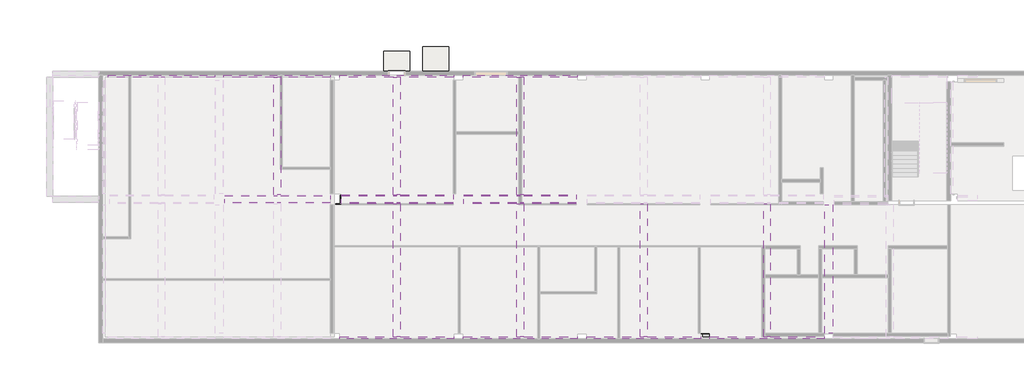
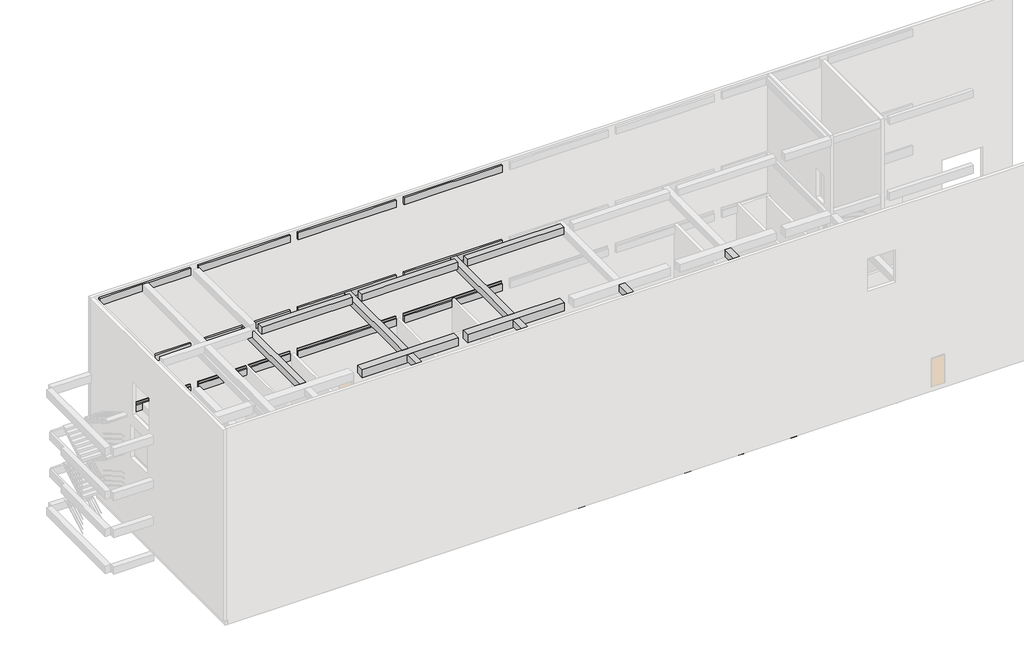
# One storey, part 3 of 5: 54 beams, 2 slabs.
"""IFC4 building model written with IfcOpenShell, lengths in millimetres."""

from ifc_helpers import new_model, si_unit, frame, origin, place, context, project, spatial, polyline, outline, extrude, faceted_brep, element, save

model = new_model("IFC4")

# Units and contexts
model_context = context("Model", 3, world=origin())
ifc_project = project(units=[si_unit("LENGTHUNIT", "METRE", prefix="MILLI")], contexts=[model_context])

# Site, building, storey
site = spatial("IfcSite", under=ifc_project)
building = spatial("IfcBuilding", under=site)
storey = spatial("IfcBuildingStorey", under=building, Name="TOC", Elevation=149.9618634)

# Beams
placement = place(None, origin())
element("IfcBeam", 1, ObjectType="RC Beam_Rectangular : H_SB_AR_S16_UG_B600xH800_1G2", at=placement, inside=storey, context=model_context, shape_type="Brep", body=[
    faceted_brep([(23300.0, 9749.5208589, -550.0381366), (23300.0, 9749.5208589, -150.0381366), (23350.0, 9749.5208589, -150.0381366), (23350.0, 9749.5208589, -0.0381366), (26775.0, 9749.5208589, -0.0381366), (27225.0, 9749.5208589, -0.0381366), (30650.0, 9749.5208589, -0.0381366), (30650.0, 9749.5208589, -150.0381366), (30700.0, 9749.5208589, -150.0381366), (30700.0, 9749.5208589, -550.0381366), (29500.0, 9749.5208589, -550.0381366), (29500.0, 9749.5208589, -650.0381366), (24500.0, 9749.5208589, -650.0381366), (24500.0, 9749.5208589, -550.0381366), (24500.0, 9149.5208589, -650.0381366), (29500.0, 9149.5208589, -650.0381366), (22750.0, 9149.5208589, -550.0381366), (23250.0, 9149.5208589, -550.0381366), (24500.0, 9149.5208589, -550.0381366), (29500.0, 9149.5208589, -550.0381366), (30750.0, 9149.5208589, -550.0381366), (31250.0, 9149.5208589, -550.0381366), (31250.0, 9149.5208589, -150.0381366), (30650.0, 9149.5208589, -150.0381366), (30650.0, 9149.5208589, -0.0381366), (27225.0, 9149.5208589, -0.0381366), (26775.0, 9149.5208589, -0.0381366), (23350.0, 9149.5208589, -0.0381366), (23350.0, 9149.5208589, -150.0381366), (22750.0, 9149.5208589, -150.0381366), (23300.0, 9199.5208589, -550.0381366), (23300.0, 9199.5208589, -150.0381366), (30700.0, 9199.5208589, -150.0381366), (30700.0, 9199.5208589, -550.0381366), (22750.0, 9199.5208589, -550.0381366), (31250.0, 9199.5208589, -550.0381366), (22750.0, 9199.5208589, -150.0381366), (31250.0, 9199.5208589, -150.0381366)], [[[0, 1, 2, 3, 4, 5, 6, 7, 8, 9, 10, 11, 12, 13]], [[14, 12, 11, 15]], [[16, 17, 18, 14, 15, 19, 20, 21, 22, 23, 24, 25, 26, 27, 28, 29]], [[30, 31, 1, 0]], [[32, 33, 9, 8]], [[13, 18, 17, 16, 34, 30, 0]], [[18, 13, 12, 14]], [[19, 10, 9, 33, 35, 21, 20]], [[10, 19, 15, 11]], [[3, 27, 26, 25, 24, 6, 5, 4]], [[31, 30, 34, 36]], [[33, 32, 37, 35]], [[28, 2, 1, 31, 36, 29]], [[2, 28, 27, 3]], [[7, 23, 22, 37, 32, 8]], [[23, 7, 6, 24]], [[36, 34, 16, 29]], [[35, 37, 22, 21]]]),
])
element("IfcBeam", 2, ObjectType="RC Beam_Rectangular : H_SB_AR_S16_UG_B450xH700_1B1", at=placement, inside=storey, context=model_context, shape_type="SweptSolid", body=[
    extrude(outline(polyline([(18775.0, 17399.5208589), (19225.0, 17399.5208589), (19225.0, 9749.5208589), (18775.0, 9749.5208589), (18775.0, 17399.5208589)])), frame((0.0, 0.0, -550.0381366), z_axis=(0.0, 0.0, 1.0), x_axis=(1.0, 0.0, 0.0)), (0.0, 0.0, 1.0), 550.0),
])
element("IfcBeam", 3, ObjectType="RC Beam_Rectangular : H_SB_AR_S16_UG_B450xH700_1B1", at=placement, inside=storey, context=model_context, shape_type="SweptSolid", body=[
    extrude(outline(polyline([(26775.0, 17399.5208589), (27225.0, 17399.5208589), (27225.0, 9749.5208589), (26775.0, 9749.5208589), (26775.0, 17399.5208589)])), frame((0.0, 0.0, -550.0381366), z_axis=(0.0, 0.0, 1.0), x_axis=(1.0, 0.0, 0.0)), (0.0, 0.0, 1.0), 550.0),
])
element("IfcBeam", 4, ObjectType="RC Beam_Rectangular : H_SB_AR_S16_UG_B500xH700_1G1", at=placement, inside=storey, context=model_context, shape_type="SweptSolid", body=[
    extrude(outline(polyline([(9799.5208589, -550.0381366), (9799.5208589, -150.0381366), (9849.5208589, -150.0381366), (9849.5208589, -0.0381366), (17199.5208589, -0.0381366), (17199.5208589, -550.0381366), (9799.5208589, -550.0381366)])), frame((30750.0, 0.0, 0.0), z_axis=(1.0, 0.0, 0.0), x_axis=(0.0, 1.0, 0.0)), (0.0, 0.0, 1.0), 500.0),
])
element("IfcBeam", 5, ObjectType="RC Beam_Rectangular : H_SB_AR_S16_UG_B500xH700_1G1", at=placement, inside=storey, context=model_context, shape_type="SweptSolid", body=[
    extrude(outline(polyline([(17199.5208589, -0.0381366), (17199.5208589, -550.0381366), (9799.5208589, -550.0381366), (9799.5208589, -150.0381366), (9849.5208589, -150.0381366), (9849.5208589, -0.0381366), (17199.5208589, -0.0381366)])), frame((22750.0, 0.0, 0.0), z_axis=(1.0, 0.0, 0.0), x_axis=(0.0, 1.0, 0.0)), (0.0, 0.0, 1.0), 500.0),
])
element("IfcBeam", 6, ObjectType="RC Beam_Rectangular : H_SB_AR_S16_UG_B500xH700_1G1", at=placement, inside=storey, context=model_context, shape_type="Brep", body=[
    faceted_brep([(23250.0, 9149.5208589, -550.0381366), (22750.0, 9149.5208589, -550.0381366), (22750.0, 9149.5208589, -150.0381366), (22750.0, 9149.5208589, -0.0381366), (23250.0, 9149.5208589, -0.0381366), (22750.0, 799.5208589, -550.0381366), (22750.0, 799.5208589, -0.0381366), (23250.0, 799.5208589, -550.0381366), (23250.0, 799.5208589, -0.0381366)], [[[0, 1, 2, 3, 4]], [[5, 6, 3, 2, 1]], [[1, 0, 7, 5]], [[8, 7, 0, 4]], [[5, 7, 8, 6]], [[3, 6, 8, 4]]]),
])
element("IfcBeam", 7, ObjectType="RC Beam_Rectangular : H_SB_AR_S16_UG_B500xH700_1G1", at=placement, inside=storey, context=model_context, shape_type="Brep", body=[
    faceted_brep([(30750.0, 799.5208589, -550.0381366), (30750.0, 799.5208589, -0.0381366), (30750.0, 9149.5208589, -0.0381366), (30750.0, 9149.5208589, -550.0381366), (31250.0, 799.5208589, -550.0381366), (31250.0, 9149.5208589, -550.0381366), (31250.0, 799.5208589, -0.0381366), (31250.0, 9149.5208589, -150.0381366), (31250.0, 9149.5208589, -0.0381366)], [[[0, 1, 2, 3]], [[4, 0, 3, 5]], [[6, 4, 5, 7, 8]], [[0, 4, 6, 1]], [[2, 1, 6, 8]], [[5, 3, 2, 8, 7]]]),
])
element("IfcBeam", 8, ObjectType="RC Beam_Rectangular : H_SB_AR_S16_UG_B500xH700_1G1", at=placement, inside=storey, context=model_context, shape_type="Brep", body=[
    faceted_brep([(39249.6103984, 9148.7405199, -550.0381366), (38749.610707, 9149.2960751, -550.0381366), (38749.610707, 9149.2960751, -0.0381366), (39249.6103984, 9148.7405199, -0.0381366), (39240.3344102, 800.351107, 149.9618634), (38740.3341015, 800.351107, 149.9618634), (38740.333179, 799.5208589, 149.9618634), (39240.3334877, 799.5208589, 149.9618634), (38740.333179, 799.5208589, -550.0381366), (38740.3341015, 800.351107, -0.0381366), (39240.1112654, 599.5208589, -550.0381366), (38850.0, 599.5208589, -550.0381366), (38850.0, 799.5208589, -550.0381366), (39240.3344102, 800.351107, -0.0381366), (39240.3334877, 799.5208589, -150.0381366), (39240.1112654, 599.5208589, -150.0381366), (38850.0, 799.5208589, -150.0381366), (38850.0, 599.5208589, -150.0381366)], [[[0, 1, 2, 3]], [[4, 5, 6, 7]], [[8, 6, 5, 9, 2, 1]], [[1, 0, 10, 11, 12, 8]], [[3, 13, 4, 7, 14, 15, 10, 0]], [[8, 12, 16, 14, 7, 6]], [[2, 9, 13, 3]], [[5, 4, 13, 9]], [[11, 10, 15, 17]], [[14, 16, 17, 15]], [[16, 12, 11, 17]]]),
])
element("IfcBeam", 9, ObjectType="RC Beam_Rectangular : H_SB_AR_S16_UG_B500xH700_1G1", at=placement, inside=storey, context=model_context, shape_type="Brep", body=[
    faceted_brep([(46750.0, 799.5208589, -550.0381366), (46750.0, 799.5208589, -0.0381366), (46750.0, 9149.5208589, -0.0381366), (46750.0, 9149.5208589, -550.0381366), (47250.0, 799.5208589, -550.0381366), (47250.0, 9149.5208589, -550.0381366), (47250.0, 799.5208589, -0.0381366), (47250.0, 9149.5208589, -150.0381366), (47250.0, 9149.5208589, -0.0381366)], [[[0, 1, 2, 3]], [[4, 0, 3, 5]], [[6, 4, 5, 7, 8]], [[0, 4, 6, 1]], [[2, 1, 6, 8]], [[2, 8, 7, 5, 3]]]),
])
element("IfcBeam", 10, ObjectType="RC Beam_Rectangular : H_SB_AR_S16_UG_B450xH700_1B1A", at=placement, inside=storey, context=model_context, shape_type="SweptSolid", body=[
    extrude(outline(polyline([(43225.0, 599.5208589), (42775.0, 599.5208589), (42775.0, 9149.5208589), (43225.0, 9149.5208589), (43225.0, 599.5208589)])), frame((0.0, 0.0, -550.0381366), z_axis=(0.0, 0.0, 1.0), x_axis=(1.0, 0.0, 0.0)), (0.0, 0.0, 1.0), 550.0),
])
element("IfcBeam", 11, ObjectType="RC Beam_Rectangular : H_SB_AR_S16_UG_B450xH700_1B1A", at=placement, inside=storey, context=model_context, shape_type="SweptSolid", body=[
    extrude(outline(polyline([(35225.0, 599.5208589), (34775.0, 599.5208589), (34775.0, 9149.5208589), (35225.0, 9149.5208589), (35225.0, 599.5208589)])), frame((0.0, 0.0, -550.0381366), z_axis=(0.0, 0.0, 1.0), x_axis=(1.0, 0.0, 0.0)), (0.0, 0.0, 1.0), 550.0),
])
element("IfcBeam", 12, ObjectType="RC Beam_Rectangular : H_SB_AR_S16_UG_B450xH700_1B1A", at=placement, inside=storey, context=model_context, shape_type="SweptSolid", body=[
    extrude(outline(polyline([(27225.0, 599.5208589), (26775.0, 599.5208589), (26775.0, 9149.5208589), (27225.0, 9149.5208589), (27225.0, 599.5208589)])), frame((0.0, 0.0, -550.0381366), z_axis=(0.0, 0.0, 1.0), x_axis=(1.0, 0.0, 0.0)), (0.0, 0.0, 1.0), 550.0),
])
element("IfcBeam", 13, ObjectType="RC Beam_Rectangular : H_SB_AR_S16_UG_B450xH700_1B1A", at=placement, inside=storey, context=model_context, shape_type="SweptSolid", body=[
    extrude(outline(polyline([(19225.0, 599.5208589), (18775.0, 599.5208589), (18775.0, 9149.5208589), (19225.0, 9149.5208589), (19225.0, 599.5208589)])), frame((0.0, 0.0, -550.0381366), z_axis=(0.0, 0.0, 1.0), x_axis=(1.0, 0.0, 0.0)), (0.0, 0.0, 1.0), 550.0),
])
element("IfcBeam", 14, ObjectType="RC Beam_Rectangular : H_SB_AR_S16_AG_B400xH700_3WG1", at=placement, inside=storey, context=model_context, shape_type="Brep", body=[
    faceted_brep([(300.0, 17499.5208589, 5949.9618634), (7200.0, 17499.5208589, 5949.9618634), (7200.0, 17549.5208589, 5949.9618634), (300.0, 17549.5208589, 5949.9618634), (300.0, 17399.5208589, 5799.9618634), (300.0, 17399.5208589, 5249.9618634), (3525.0, 17399.5208589, 5249.9618634), (3975.0, 17399.5208589, 5249.9618634), (7200.0, 17399.5208589, 5249.9618634), (7200.0, 17399.5208589, 5799.9618634), (3975.0, 17399.5208589, 5799.9618634), (3525.0, 17399.5208589, 5799.9618634), (300.0, 17549.5208589, 5249.9618634), (7200.0, 17549.5208589, 5249.9618634), (300.0, 17499.5208589, 5799.9618634), (7200.0, 17499.5208589, 5799.9618634)], [[[0, 1, 2, 3]], [[4, 5, 6, 7, 8, 9, 10, 11]], [[8, 7, 6, 5, 12, 13]], [[14, 4, 11, 10, 9, 15]], [[0, 14, 15, 1]], [[5, 4, 14, 0, 3, 12]], [[9, 8, 13, 2, 1, 15]], [[3, 2, 13, 12]]]),
])
element("IfcBeam", 15, ObjectType="RC Beam_Rectangular : H_SB_AR_S16_AG_B400xH700_3WG1", at=placement, inside=storey, context=model_context, shape_type="Brep", body=[
    faceted_brep([(7800.0, 17499.5208589, 5949.9618634), (14700.0, 17499.5208589, 5949.9618634), (14700.0, 17549.5208589, 5949.9618634), (7800.0, 17549.5208589, 5949.9618634), (7800.0, 17399.5208589, 5799.9618634), (7800.0, 17399.5208589, 5249.9618634), (11050.0, 17399.5208589, 5249.9618634), (11500.0, 17399.5208589, 5249.9618634), (14700.0, 17399.5208589, 5249.9618634), (14700.0, 17399.5208589, 5799.9618634), (11500.0, 17399.5208589, 5799.9618634), (11050.0, 17399.5208589, 5799.9618634), (7800.0, 17549.5208589, 5249.9618634), (14700.0, 17549.5208589, 5249.9618634), (7800.0, 17499.5208589, 5799.9618634), (14700.0, 17499.5208589, 5799.9618634)], [[[0, 1, 2, 3]], [[4, 5, 6, 7, 8, 9, 10, 11]], [[8, 7, 6, 5, 12, 13]], [[14, 4, 11, 10, 9, 15]], [[0, 14, 15, 1]], [[5, 4, 14, 0, 3, 12]], [[9, 8, 13, 2, 1, 15]], [[3, 2, 13, 12]]]),
])
element("IfcBeam", 16, ObjectType="RC Beam_Rectangular : H_SB_AR_S16_AG_B400xH700_3WG1", at=placement, inside=storey, context=model_context, shape_type="Brep", body=[
    faceted_brep([(15300.0, 17499.5208589, 5949.9618634), (22700.0, 17499.5208589, 5949.9618634), (22700.0, 17549.5208589, 5949.9618634), (15300.0, 17549.5208589, 5949.9618634), (15300.0, 17399.5208589, 5799.9618634), (15300.0, 17399.5208589, 5249.9618634), (18800.0, 17399.5208589, 5249.9618634), (19250.0, 17399.5208589, 5249.9618634), (22700.0, 17399.5208589, 5249.9618634), (22700.0, 17399.5208589, 5799.9618634), (19250.0, 17399.5208589, 5799.9618634), (18800.0, 17399.5208589, 5799.9618634), (15300.0, 17549.5208589, 5249.9618634), (22700.0, 17549.5208589, 5249.9618634), (15300.0, 17499.5208589, 5799.9618634), (22700.0, 17499.5208589, 5799.9618634)], [[[0, 1, 2, 3]], [[4, 5, 6, 7, 8, 9, 10, 11]], [[8, 7, 6, 5, 12, 13]], [[14, 4, 11, 10, 9, 15]], [[0, 14, 15, 1]], [[5, 4, 14, 0, 3, 12]], [[9, 8, 13, 2, 1, 15]], [[3, 2, 13, 12]]]),
])
element("IfcBeam", 17, ObjectType="RC Beam_Rectangular : H_SB_AR_S16_AG_B400xH700_3WG1", at=placement, inside=storey, context=model_context, shape_type="Brep", body=[
    faceted_brep([(23300.0, 17499.5208589, 5949.9618634), (30700.0, 17499.5208589, 5949.9618634), (30700.0, 17549.5208589, 5949.9618634), (23300.0, 17549.5208589, 5949.9618634), (23300.0, 17399.5208589, 5799.9618634), (23300.0, 17399.5208589, 5249.9618634), (26775.0, 17399.5208589, 5249.9618634), (27225.0, 17399.5208589, 5249.9618634), (30700.0, 17399.5208589, 5249.9618634), (30700.0, 17399.5208589, 5799.9618634), (27225.0, 17399.5208589, 5799.9618634), (26775.0, 17399.5208589, 5799.9618634), (23300.0, 17549.5208589, 5249.9618634), (30700.0, 17549.5208589, 5249.9618634), (23300.0, 17499.5208589, 5799.9618634), (30700.0, 17499.5208589, 5799.9618634)], [[[0, 1, 2, 3]], [[4, 5, 6, 7, 8, 9, 10, 11]], [[8, 7, 6, 5, 12, 13]], [[14, 4, 11, 10, 9, 15]], [[0, 14, 15, 1]], [[5, 4, 14, 0, 3, 12]], [[9, 8, 13, 2, 1, 15]], [[3, 2, 13, 12]]]),
])
element("IfcBeam", 18, ObjectType="RC Beam_Rectangular : H_SB_AR_S16_AG_B400xH700_3WG1", at=placement, inside=storey, context=model_context, shape_type="Brep", body=[
    faceted_brep([(22700.0, 449.5208589, 5949.9618634), (22700.0, 499.5208589, 5949.9618634), (15300.0, 499.5208589, 5949.9618634), (15300.0, 449.5208589, 5949.9618634), (22700.0, 599.5208589, 5249.9618634), (22700.0, 449.5208589, 5249.9618634), (15300.0, 449.5208589, 5249.9618634), (15300.0, 599.5208589, 5249.9618634), (18785.0, 599.5208589, 5249.9618634), (19235.0, 599.5208589, 5249.9618634), (22700.0, 599.5208589, 5799.9618634), (15300.0, 599.5208589, 5799.9618634), (18785.0, 599.5208589, 5799.9618634), (19235.0, 599.5208589, 5799.9618634), (22700.0, 499.5208589, 5799.9618634), (15300.0, 499.5208589, 5799.9618634)], [[[0, 1, 2, 3]], [[4, 5, 6, 7, 8, 9]], [[10, 4, 9, 8, 7, 11, 12, 13]], [[5, 0, 3, 6]], [[14, 10, 13, 12, 11, 15]], [[1, 14, 15, 2]], [[1, 0, 5, 4, 10, 14]], [[3, 2, 15, 11, 7, 6]]]),
])
element("IfcBeam", 19, ObjectType="RC Beam_Rectangular : H_SB_AR_S16_AG_B400xH700_3WG1", at=placement, inside=storey, context=model_context, shape_type="Brep", body=[
    faceted_brep([(30700.0, 449.5208589, 5949.9618634), (30700.0, 499.5208589, 5949.9618634), (23300.0, 499.5208589, 5949.9618634), (23300.0, 449.5208589, 5949.9618634), (30700.0, 599.5208589, 5249.9618634), (30700.0, 449.5208589, 5249.9618634), (23300.0, 449.5208589, 5249.9618634), (23300.0, 599.5208589, 5249.9618634), (26785.0, 599.5208589, 5249.9618634), (27235.0, 599.5208589, 5249.9618634), (30700.0, 599.5208589, 5799.9618634), (23300.0, 599.5208589, 5799.9618634), (26785.0, 599.5208589, 5799.9618634), (27235.0, 599.5208589, 5799.9618634), (30700.0, 499.5208589, 5799.9618634), (23300.0, 499.5208589, 5799.9618634)], [[[0, 1, 2, 3]], [[4, 5, 6, 7, 8, 9]], [[10, 4, 9, 8, 7, 11, 12, 13]], [[5, 0, 3, 6]], [[14, 10, 13, 12, 11, 15]], [[1, 14, 15, 2]], [[1, 0, 5, 4, 10, 14]], [[3, 2, 15, 11, 7, 6]]]),
])
element("IfcBeam", 20, ObjectType="RC Beam_Rectangular : H_SB_AR_S16_AG_B400xH700_3WG1", at=placement, inside=storey, context=model_context, shape_type="Brep", body=[
    faceted_brep([(38700.0, 449.5208589, 5949.9618634), (38700.0, 499.5208589, 5949.9618634), (31300.0, 499.5208589, 5949.9618634), (31300.0, 449.5208589, 5949.9618634), (38700.0, 599.5208589, 5249.9618634), (38700.0, 449.5208589, 5249.9618634), (31300.0, 449.5208589, 5249.9618634), (31300.0, 599.5208589, 5249.9618634), (34785.0, 599.5208589, 5249.9618634), (35235.0, 599.5208589, 5249.9618634), (38700.0, 599.5208589, 5799.9618634), (31300.0, 599.5208589, 5799.9618634), (34785.0, 599.5208589, 5799.9618634), (35235.0, 599.5208589, 5799.9618634), (38700.0, 499.5208589, 5799.9618634), (31300.0, 499.5208589, 5799.9618634)], [[[0, 1, 2, 3]], [[4, 5, 6, 7, 8, 9]], [[10, 4, 9, 8, 7, 11, 12, 13]], [[5, 0, 3, 6]], [[14, 10, 13, 12, 11, 15]], [[1, 14, 15, 2]], [[1, 0, 5, 4, 10, 14]], [[3, 2, 15, 11, 7, 6]]]),
])
element("IfcBeam", 21, ObjectType="RC Beam_Rectangular : H_SB_AR_S16_AG_B400xH700_3WG1", at=placement, inside=storey, context=model_context, shape_type="Brep", body=[
    faceted_brep([(46700.0, 449.5208589, 5949.9618634), (46700.0, 499.5208589, 5949.9618634), (39300.0, 499.5208589, 5949.9618634), (39300.0, 449.5208589, 5949.9618634), (46700.0, 599.5208589, 5249.9618634), (46700.0, 449.5208589, 5249.9618634), (39300.0, 449.5208589, 5249.9618634), (39300.0, 599.5208589, 5249.9618634), (42785.0, 599.5208589, 5249.9618634), (43235.0, 599.5208589, 5249.9618634), (46700.0, 599.5208589, 5799.9618634), (39300.0, 599.5208589, 5799.9618634), (42785.0, 599.5208589, 5799.9618634), (43235.0, 599.5208589, 5799.9618634), (46700.0, 499.5208589, 5799.9618634), (39300.0, 499.5208589, 5799.9618634)], [[[0, 1, 2, 3]], [[4, 5, 6, 7, 8, 9]], [[10, 4, 9, 8, 7, 11, 12, 13]], [[5, 0, 3, 6]], [[14, 10, 13, 12, 11, 15]], [[1, 14, 15, 2]], [[1, 0, 5, 4, 10, 14]], [[3, 2, 15, 11, 7, 6]]]),
])
element("IfcBeam", 22, ObjectType="RC Beam_Rectangular : H_SB_AR_S16_AG_B600xH800_3G2", at=placement, inside=storey, context=model_context, shape_type="Brep", body=[
    faceted_brep([(15400.0, 9199.5208589, 5149.9618634), (22650.0, 9199.5208589, 5149.9618634), (22650.0, 9199.5208589, 5799.9618634), (19235.0, 9199.5208589, 5799.9618634), (18785.0, 9199.5208589, 5799.9618634), (15400.0, 9199.5208589, 5799.9618634), (15400.0, 9799.5208589, 5149.9618634), (22650.0, 9799.5208589, 5149.9618634), (15400.0, 9799.5208589, 5799.9618634), (18800.0, 9799.5208589, 5799.9618634), (19250.0, 9799.5208589, 5799.9618634), (22650.0, 9799.5208589, 5799.9618634)], [[[0, 1, 2, 3, 4, 5]], [[1, 0, 6, 7]], [[7, 6, 8, 9, 10, 11]], [[5, 4, 3, 2, 11, 10, 9, 8]], [[1, 7, 11, 2]], [[6, 0, 5, 8]]]),
])
element("IfcBeam", 23, ObjectType="RC Beam_Rectangular : H_SB_AR_S16_AG_B600xH800_3G2", at=placement, inside=storey, context=model_context, shape_type="Brep", body=[
    faceted_brep([(23350.0, 9199.5208589, 5149.9618634), (30650.0, 9199.5208589, 5149.9618634), (30650.0, 9199.5208589, 5799.9618634), (27235.0, 9199.5208589, 5799.9618634), (26785.0, 9199.5208589, 5799.9618634), (23350.0, 9199.5208589, 5799.9618634), (23350.0, 9799.5208589, 5149.9618634), (30650.0, 9799.5208589, 5149.9618634), (23350.0, 9799.5208589, 5799.9618634), (26775.0, 9799.5208589, 5799.9618634), (27225.0, 9799.5208589, 5799.9618634), (30650.0, 9799.5208589, 5799.9618634)], [[[0, 1, 2, 3, 4, 5]], [[1, 0, 6, 7]], [[7, 6, 8, 9, 10, 11]], [[5, 4, 3, 2, 11, 10, 9, 8]], [[6, 0, 5, 8]], [[1, 7, 11, 2]]]),
])
element("IfcBeam", 24, ObjectType="RC Beam_Rectangular : H_SB_AR_S16_AG_B4500xH700_3G1", at=placement, inside=storey, context=model_context, shape_type="SweptSolid", body=[
    extrude(outline(polyline([(46750.0, 799.5208589), (46750.0, 9149.5208589), (47250.0, 9149.5208589), (47250.0, 799.5208589), (46750.0, 799.5208589)])), frame((0.0, 0.0, 5249.9618634), z_axis=(0.0, 0.0, 1.0), x_axis=(1.0, 0.0, 0.0)), (0.0, 0.0, 1.0), 550.0),
])
element("IfcBeam", 25, ObjectType="RC Beam_Rectangular : H_SB_AR_S16_AG_B400xH700_3WG1", at=placement, inside=storey, context=model_context, shape_type="Brep", body=[
    faceted_brep([(300.0, 17399.5208589, 9269.9618634), (300.0, 17399.5208589, 8749.9618634), (3525.0, 17399.5208589, 8749.9618634), (3975.0, 17399.5208589, 8749.9618634), (7200.0, 17399.5208589, 8749.9618634), (7200.0, 17399.5208589, 9269.9618634), (3975.0, 17399.5208589, 9269.9618634), (3525.0, 17399.5208589, 9269.9618634), (300.0, 17549.5208589, 8749.9618634), (7200.0, 17549.5208589, 8749.9618634), (300.0, 17549.5208589, 9269.9618634), (7200.0, 17549.5208589, 9269.9618634)], [[[0, 1, 2, 3, 4, 5, 6, 7]], [[4, 3, 2, 1, 8, 9]], [[10, 0, 7, 6, 5, 11]], [[1, 0, 10, 8]], [[5, 4, 9, 11]], [[9, 8, 10, 11]]]),
])
element("IfcBeam", 26, ObjectType="RC Beam_Rectangular : H_SB_AR_S16_AG_B400xH700_3WG1", at=placement, inside=storey, context=model_context, shape_type="Brep", body=[
    faceted_brep([(7800.0, 17399.5208589, 9269.9618634), (7800.0, 17399.5208589, 8749.9618634), (11025.0, 17399.5208589, 8749.9618634), (11475.0, 17399.5208589, 8749.9618634), (14700.0, 17399.5208589, 8749.9618634), (14700.0, 17399.5208589, 9269.9618634), (11475.0, 17399.5208589, 9269.9618634), (11025.0, 17399.5208589, 9269.9618634), (7800.0, 17549.5208589, 8749.9618634), (14700.0, 17549.5208589, 8749.9618634), (7800.0, 17549.5208589, 9269.9618634), (14700.0, 17549.5208589, 9269.9618634)], [[[0, 1, 2, 3, 4, 5, 6, 7]], [[4, 3, 2, 1, 8, 9]], [[10, 0, 7, 6, 5, 11]], [[1, 0, 10, 8]], [[5, 4, 9, 11]], [[9, 8, 10, 11]]]),
])
element("IfcBeam", 27, ObjectType="RC Beam_Rectangular : H_SB_AR_S16_AG_B400xH700_3WG1", at=placement, inside=storey, context=model_context, shape_type="Brep", body=[
    faceted_brep([(15300.0, 17399.5208589, 9269.9618634), (15300.0, 17399.5208589, 8749.9618634), (18775.0, 17399.5208589, 8749.9618634), (19225.0, 17399.5208589, 8749.9618634), (22700.0, 17399.5208589, 8749.9618634), (22700.0, 17399.5208589, 9269.9618634), (19225.0, 17399.5208589, 9269.9618634), (18775.0, 17399.5208589, 9269.9618634), (15300.0, 17549.5208589, 8749.9618634), (22700.0, 17549.5208589, 8749.9618634), (15300.0, 17549.5208589, 9269.9618634), (22700.0, 17549.5208589, 9269.9618634)], [[[0, 1, 2, 3, 4, 5, 6, 7]], [[4, 3, 2, 1, 8, 9]], [[10, 0, 7, 6, 5, 11]], [[1, 0, 10, 8]], [[5, 4, 9, 11]], [[9, 8, 10, 11]]]),
])
element("IfcBeam", 28, ObjectType="RC Beam_Rectangular : H_SB_AR_S16_AG_B400xH700_3WG1", at=placement, inside=storey, context=model_context, shape_type="Brep", body=[
    faceted_brep([(23300.0, 17399.5208589, 9269.9618634), (23300.0, 17399.5208589, 8749.9618634), (26775.0, 17399.5208589, 8749.9618634), (27225.0, 17399.5208589, 8749.9618634), (30700.0, 17399.5208589, 8749.9618634), (30700.0, 17399.5208589, 9269.9618634), (27225.0, 17399.5208589, 9269.9618634), (26775.0, 17399.5208589, 9269.9618634), (23300.0, 17549.5208589, 8749.9618634), (30700.0, 17549.5208589, 8749.9618634), (23300.0, 17549.5208589, 9269.9618634), (30700.0, 17549.5208589, 9269.9618634)], [[[0, 1, 2, 3, 4, 5, 6, 7]], [[4, 3, 2, 1, 8, 9]], [[10, 0, 7, 6, 5, 11]], [[1, 0, 10, 8]], [[5, 4, 9, 11]], [[9, 8, 10, 11]]]),
])
element("IfcBeam", 29, ObjectType="RC Beam_Rectangular : H_SB_AR_S16_AG_B400xH700_3WG1", at=placement, inside=storey, context=model_context, shape_type="Brep", body=[
    faceted_brep([(22700.0, 599.5208589, 8749.9618634), (22700.0, 449.5208589, 8749.9618634), (15300.0, 449.5208589, 8749.9618634), (15300.0, 599.5208589, 8749.9618634), (18775.0, 599.5208589, 8749.9618634), (19225.0, 599.5208589, 8749.9618634), (22700.0, 599.5208589, 9269.9618634), (15300.0, 599.5208589, 9269.9618634), (18775.0, 599.5208589, 9269.9618634), (19225.0, 599.5208589, 9269.9618634), (22700.0, 449.5208589, 9269.9618634), (15300.0, 449.5208589, 9269.9618634)], [[[0, 1, 2, 3, 4, 5]], [[6, 0, 5, 4, 3, 7, 8, 9]], [[1, 10, 11, 2]], [[10, 6, 9, 8, 7, 11]], [[1, 0, 6, 10]], [[3, 2, 11, 7]]]),
])
element("IfcBeam", 30, ObjectType="RC Beam_Rectangular : H_SB_AR_S16_AG_B400xH700_3WG1", at=placement, inside=storey, context=model_context, shape_type="Brep", body=[
    faceted_brep([(30700.0, 599.5208589, 8749.9618634), (30700.0, 449.5208589, 8749.9618634), (23300.0, 449.5208589, 8749.9618634), (23300.0, 599.5208589, 8749.9618634), (26775.0, 599.5208589, 8749.9618634), (27225.0, 599.5208589, 8749.9618634), (30700.0, 599.5208589, 9269.9618634), (23300.0, 599.5208589, 9269.9618634), (26775.0, 599.5208589, 9269.9618634), (27225.0, 599.5208589, 9269.9618634), (30700.0, 449.5208589, 9269.9618634), (23300.0, 449.5208589, 9269.9618634)], [[[0, 1, 2, 3, 4, 5]], [[6, 0, 5, 4, 3, 7, 8, 9]], [[1, 10, 11, 2]], [[10, 6, 9, 8, 7, 11]], [[1, 0, 6, 10]], [[3, 2, 11, 7]]]),
])
element("IfcBeam", 31, ObjectType="RC Beam_Rectangular : H_SB_AR_S16_AG_B400xH700_3WG1", at=placement, inside=storey, context=model_context, shape_type="Brep", body=[
    faceted_brep([(38700.0, 599.5208589, 8749.9618634), (38700.0, 449.5208589, 8749.9618634), (31300.0, 449.5208589, 8749.9618634), (31300.0, 599.5208589, 8749.9618634), (34775.0, 599.5208589, 8749.9618634), (35225.0, 599.5208589, 8749.9618634), (38700.0, 599.5208589, 9269.9618634), (31300.0, 599.5208589, 9269.9618634), (34775.0, 599.5208589, 9269.9618634), (35225.0, 599.5208589, 9269.9618634), (38700.0, 449.5208589, 9269.9618634), (31300.0, 449.5208589, 9269.9618634)], [[[0, 1, 2, 3, 4, 5]], [[6, 0, 5, 4, 3, 7, 8, 9]], [[1, 10, 11, 2]], [[10, 6, 9, 8, 7, 11]], [[1, 0, 6, 10]], [[3, 2, 11, 7]]]),
])
element("IfcBeam", 32, ObjectType="RC Beam_Rectangular : H_SB_AR_S16_AG_B400xH700_3WG1", at=placement, inside=storey, context=model_context, shape_type="Brep", body=[
    faceted_brep([(46700.0, 599.5208589, 8749.9618634), (46700.0, 449.5208589, 8749.9618634), (39300.0, 449.5208589, 8749.9618634), (39300.0, 599.5208589, 8749.9618634), (42775.0, 599.5208589, 8749.9618634), (43225.0, 599.5208589, 8749.9618634), (46700.0, 599.5208589, 9269.9618634), (39300.0, 599.5208589, 9269.9618634), (42775.0, 599.5208589, 9269.9618634), (43225.0, 599.5208589, 9269.9618634), (46700.0, 449.5208589, 9269.9618634), (39300.0, 449.5208589, 9269.9618634)], [[[0, 1, 2, 3, 4, 5]], [[6, 0, 5, 4, 3, 7, 8, 9]], [[1, 10, 11, 2]], [[10, 6, 9, 8, 7, 11]], [[1, 0, 6, 10]], [[3, 2, 11, 7]]]),
])
element("IfcBeam", 33, ObjectType="RC Beam_Rectangular : H_SB_AR_S16_AG_B600xH800_3G2", at=placement, inside=storey, context=model_context, shape_type="Brep", body=[
    faceted_brep([(15400.0, 9199.5208589, 8649.9618634), (22650.0, 9199.5208589, 8649.9618634), (22650.0, 9199.5208589, 9269.9618634), (19225.0, 9199.5208589, 9269.9618634), (18775.0, 9199.5208589, 9269.9618634), (15400.0, 9199.5208589, 9269.9618634), (15400.0, 9799.5208589, 8649.9618634), (22650.0, 9799.5208589, 8649.9618634), (15400.0, 9799.5208589, 9269.9618634), (18775.0, 9799.5208589, 9269.9618634), (19225.0, 9799.5208589, 9269.9618634), (22650.0, 9799.5208589, 9269.9618634)], [[[0, 1, 2, 3, 4, 5]], [[1, 0, 6, 7]], [[7, 6, 8, 9, 10, 11]], [[5, 4, 3, 2, 11, 10, 9, 8]], [[1, 7, 11, 2]], [[6, 0, 5, 8]]]),
])
element("IfcBeam", 34, ObjectType="RC Beam_Rectangular : H_SB_AR_S16_AG_B600xH800_3G2", at=placement, inside=storey, context=model_context, shape_type="Brep", body=[
    faceted_brep([(23350.0, 9199.5208589, 8649.9618634), (30650.0, 9199.5208589, 8649.9618634), (30650.0, 9199.5208589, 9269.9618634), (27225.0, 9199.5208589, 9269.9618634), (26775.0, 9199.5208589, 9269.9618634), (23350.0, 9199.5208589, 9269.9618634), (23350.0, 9799.5208589, 8649.9618634), (30650.0, 9799.5208589, 8649.9618634), (23350.0, 9799.5208589, 9269.9618634), (26775.0, 9799.5208589, 9269.9618634), (27225.0, 9799.5208589, 9269.9618634), (30650.0, 9799.5208589, 9269.9618634)], [[[0, 1, 2, 3, 4, 5]], [[1, 0, 6, 7]], [[7, 6, 8, 9, 10, 11]], [[5, 4, 3, 2, 11, 10, 9, 8]], [[6, 0, 5, 8]], [[1, 7, 11, 2]]]),
])
element("IfcBeam", 35, ObjectType="RC Beam_Rectangular : H_SB_AR_S16_AG_B450xH700_3B1", at=placement, inside=storey, context=model_context, shape_type="SweptSolid", body=[
    extrude(outline(polyline([(11025.0, 17399.5208589), (11475.0, 17399.5208589), (11475.0, 9799.5208589), (11025.0, 9799.5208589), (11025.0, 17399.5208589)])), frame((0.0, 0.0, 8749.9618634), z_axis=(0.0, 0.0, 1.0), x_axis=(1.0, 0.0, 0.0)), (0.0, 0.0, 1.0), 520.0),
])
element("IfcBeam", 36, ObjectType="RC Beam_Rectangular : H_SB_AR_S16_AG_B450xH700_3B1", at=placement, inside=storey, context=model_context, shape_type="SweptSolid", body=[
    extrude(outline(polyline([(18775.0, 17399.5208589), (19225.0, 17399.5208589), (19225.0, 9799.5208589), (18775.0, 9799.5208589), (18775.0, 17399.5208589)])), frame((0.0, 0.0, 8749.9618634), z_axis=(0.0, 0.0, 1.0), x_axis=(1.0, 0.0, 0.0)), (0.0, 0.0, 1.0), 520.0),
])
element("IfcBeam", 37, ObjectType="RC Beam_Rectangular : H_SB_AR_S16_AG_B450xH700_3B1", at=placement, inside=storey, context=model_context, shape_type="SweptSolid", body=[
    extrude(outline(polyline([(26775.0, 17399.5208589), (27225.0, 17399.5208589), (27225.0, 9799.5208589), (26775.0, 9799.5208589), (26775.0, 17399.5208589)])), frame((0.0, 0.0, 8749.9618634), z_axis=(0.0, 0.0, 1.0), x_axis=(1.0, 0.0, 0.0)), (0.0, 0.0, 1.0), 520.0),
])
element("IfcBeam", 38, ObjectType="RC Beam_Rectangular : H_SB_AR_S16_AG_B450xH700_3B1A", at=placement, inside=storey, context=model_context, shape_type="SweptSolid", body=[
    extrude(outline(polyline([(19225.0, 599.5208589), (18775.0, 599.5208589), (18775.0, 9199.5208589), (19225.0, 9199.5208589), (19225.0, 599.5208589)])), frame((0.0, 0.0, 8749.9618634), z_axis=(0.0, 0.0, 1.0), x_axis=(1.0, 0.0, 0.0)), (0.0, 0.0, 1.0), 520.0),
])
element("IfcBeam", 39, ObjectType="RC Beam_Rectangular : H_SB_AR_S16_AG_B450xH700_3B1A", at=placement, inside=storey, context=model_context, shape_type="SweptSolid", body=[
    extrude(outline(polyline([(27225.0, 599.5208589), (26775.0, 599.5208589), (26775.0, 9199.5208589), (27225.0, 9199.5208589), (27225.0, 599.5208589)])), frame((0.0, 0.0, 8749.9618634), z_axis=(0.0, 0.0, 1.0), x_axis=(1.0, 0.0, 0.0)), (0.0, 0.0, 1.0), 520.0),
])
element("IfcBeam", 40, ObjectType="RC Beam_Rectangular : H_SB_AR_S16_AG_B450xH700_3B1A", at=placement, inside=storey, context=model_context, shape_type="SweptSolid", body=[
    extrude(outline(polyline([(35225.0, 599.5208589), (34775.0, 599.5208589), (34775.0, 9199.5208589), (35225.0, 9199.5208589), (35225.0, 599.5208589)])), frame((0.0, 0.0, 8749.9618634), z_axis=(0.0, 0.0, 1.0), x_axis=(1.0, 0.0, 0.0)), (0.0, 0.0, 1.0), 520.0),
])
element("IfcBeam", 41, ObjectType="RC Beam_Rectangular : H_SB_AR_S16_AG_B450xH700_3B1A", at=placement, inside=storey, context=model_context, shape_type="SweptSolid", body=[
    extrude(outline(polyline([(43225.0, 599.5208589), (42775.0, 599.5208589), (42775.0, 9199.5208589), (43225.0, 9199.5208589), (43225.0, 599.5208589)])), frame((0.0, 0.0, 8749.9618634), z_axis=(0.0, 0.0, 1.0), x_axis=(1.0, 0.0, 0.0)), (0.0, 0.0, 1.0), 520.0),
])
element("IfcBeam", 42, ObjectType="RC Beam_Rectangular : H_SB_AR_S16_AG_B400xH700_RWG1", at=placement, inside=storey, context=model_context, shape_type="Brep", body=[
    faceted_brep([(300.0, 17399.5208589, 15259.9618634), (300.0, 17399.5208589, 14709.9618634), (3525.0, 17399.5208589, 14709.9618634), (3975.0, 17399.5208589, 14709.9618634), (7200.0, 17399.5208589, 14709.9618634), (7200.0, 17399.5208589, 15259.9618634), (3975.0, 17399.5208589, 15259.9618634), (3525.0, 17399.5208589, 15259.9618634), (300.0, 17549.5208589, 14709.9618634), (7200.0, 17549.5208589, 14709.9618634), (300.0, 17549.5208589, 15259.9618634), (7200.0, 17549.5208589, 15259.9618634)], [[[0, 1, 2, 3, 4, 5, 6, 7]], [[4, 3, 2, 1, 8, 9]], [[10, 0, 7, 6, 5, 11]], [[1, 0, 10, 8]], [[5, 4, 9, 11]], [[9, 8, 10, 11]]]),
])
element("IfcBeam", 43, ObjectType="RC Beam_Rectangular : H_SB_AR_S16_AG_B400xH700_RWG1", at=placement, inside=storey, context=model_context, shape_type="Brep", body=[
    faceted_brep([(7800.0, 17399.5208589, 15259.9618634), (7800.0, 17399.5208589, 14709.9618634), (11025.0, 17399.5208589, 14709.9618634), (11475.0, 17399.5208589, 14709.9618634), (14700.0, 17399.5208589, 14709.9618634), (14700.0, 17399.5208589, 15259.9618634), (11475.0, 17399.5208589, 15259.9618634), (11025.0, 17399.5208589, 15259.9618634), (7800.0, 17549.5208589, 14709.9618634), (14700.0, 17549.5208589, 14709.9618634), (7800.0, 17549.5208589, 15259.9618634), (14700.0, 17549.5208589, 15259.9618634)], [[[0, 1, 2, 3, 4, 5, 6, 7]], [[4, 3, 2, 1, 8, 9]], [[10, 0, 7, 6, 5, 11]], [[1, 0, 10, 8]], [[5, 4, 9, 11]], [[9, 8, 10, 11]]]),
])
element("IfcBeam", 44, ObjectType="RC Beam_Rectangular : H_SB_AR_S16_AG_B400xH700_RWG1", at=placement, inside=storey, context=model_context, shape_type="Brep", body=[
    faceted_brep([(15300.0, 17399.5208589, 15259.9618634), (15300.0, 17399.5208589, 14709.9618634), (18775.0, 17399.5208589, 14709.9618634), (19225.0, 17399.5208589, 14709.9618634), (22700.0, 17399.5208589, 14709.9618634), (22700.0, 17399.5208589, 15259.9618634), (19225.0, 17399.5208589, 15259.9618634), (18775.0, 17399.5208589, 15259.9618634), (15300.0, 17549.5208589, 14709.9618634), (22700.0, 17549.5208589, 14709.9618634), (15300.0, 17549.5208589, 15259.9618634), (22700.0, 17549.5208589, 15259.9618634)], [[[0, 1, 2, 3, 4, 5, 6, 7]], [[4, 3, 2, 1, 8, 9]], [[10, 0, 7, 6, 5, 11]], [[1, 0, 10, 8]], [[5, 4, 9, 11]], [[9, 8, 10, 11]]]),
])
element("IfcBeam", 45, ObjectType="RC Beam_Rectangular : H_SB_AR_S16_AG_B400xH700_RWG1", at=placement, inside=storey, context=model_context, shape_type="Brep", body=[
    faceted_brep([(23300.0, 17399.5208589, 15259.9618634), (23300.0, 17399.5208589, 14709.9618634), (26775.0, 17399.5208589, 14709.9618634), (27225.0, 17399.5208589, 14709.9618634), (30700.0, 17399.5208589, 14709.9618634), (30700.0, 17399.5208589, 15259.9618634), (27225.0, 17399.5208589, 15259.9618634), (26775.0, 17399.5208589, 15259.9618634), (23300.0, 17549.5208589, 14709.9618634), (30700.0, 17549.5208589, 14709.9618634), (23300.0, 17549.5208589, 15259.9618634), (30700.0, 17549.5208589, 15259.9618634)], [[[0, 1, 2, 3, 4, 5, 6, 7]], [[4, 3, 2, 1, 8, 9]], [[10, 0, 7, 6, 5, 11]], [[1, 0, 10, 8]], [[5, 4, 9, 11]], [[9, 8, 10, 11]]]),
])
element("IfcBeam", 46, ObjectType="RC Beam_Rectangular : H_SB_AR_S16_AG_B400xH700_RWG1", at=placement, inside=storey, context=model_context, shape_type="Brep", body=[
    faceted_brep([(22700.0, 599.5208589, 14709.9618634), (22700.0, 449.5208589, 14709.9618634), (15300.0, 449.5208589, 14709.9618634), (15300.0, 599.5208589, 14709.9618634), (18775.0, 599.5208589, 14709.9618634), (19225.0, 599.5208589, 14709.9618634), (22700.0, 599.5208589, 15259.9618634), (15300.0, 599.5208589, 15259.9618634), (18775.0, 599.5208589, 15259.9618634), (19225.0, 599.5208589, 15259.9618634), (22700.0, 449.5208589, 15259.9618634), (15300.0, 449.5208589, 15259.9618634)], [[[0, 1, 2, 3, 4, 5]], [[6, 0, 5, 4, 3, 7, 8, 9]], [[1, 10, 11, 2]], [[10, 6, 9, 8, 7, 11]], [[1, 0, 6, 10]], [[3, 2, 11, 7]]]),
])
element("IfcBeam", 47, ObjectType="RC Beam_Rectangular : H_SB_AR_S16_AG_B400xH700_RWG1", at=placement, inside=storey, context=model_context, shape_type="Brep", body=[
    faceted_brep([(30700.0, 599.5208589, 14709.9618634), (30700.0, 449.5208589, 14709.9618634), (23300.0, 449.5208589, 14709.9618634), (23300.0, 599.5208589, 14709.9618634), (26775.0, 599.5208589, 14709.9618634), (27225.0, 599.5208589, 14709.9618634), (30700.0, 599.5208589, 15259.9618634), (23300.0, 599.5208589, 15259.9618634), (26775.0, 599.5208589, 15259.9618634), (27225.0, 599.5208589, 15259.9618634), (30700.0, 449.5208589, 15259.9618634), (23300.0, 449.5208589, 15259.9618634)], [[[0, 1, 2, 3, 4, 5]], [[6, 0, 5, 4, 3, 7, 8, 9]], [[1, 10, 11, 2]], [[10, 6, 9, 8, 7, 11]], [[1, 0, 6, 10]], [[3, 2, 11, 7]]]),
])
element("IfcBeam", 48, ObjectType="RC Beam_Rectangular : H_SB_AR_S16_AG_B400xH700_RWG1", at=placement, inside=storey, context=model_context, shape_type="Brep", body=[
    faceted_brep([(38700.0, 599.5208589, 14709.9618634), (38700.0, 449.5208589, 14709.9618634), (31300.0, 449.5208589, 14709.9618634), (31300.0, 599.5208589, 14709.9618634), (34775.0, 599.5208589, 14709.9618634), (35225.0, 599.5208589, 14709.9618634), (38700.0, 599.5208589, 15259.9618634), (31300.0, 599.5208589, 15259.9618634), (34775.0, 599.5208589, 15259.9618634), (35225.0, 599.5208589, 15259.9618634), (38700.0, 449.5208589, 15259.9618634), (31300.0, 449.5208589, 15259.9618634)], [[[0, 1, 2, 3, 4, 5]], [[6, 0, 5, 4, 3, 7, 8, 9]], [[1, 10, 11, 2]], [[10, 6, 9, 8, 7, 11]], [[1, 0, 6, 10]], [[3, 2, 11, 7]]]),
])
element("IfcBeam", 49, ObjectType="RC Beam_Rectangular : H_SB_AR_S16_AG_B400xH700_RWG1", at=placement, inside=storey, context=model_context, shape_type="Brep", body=[
    faceted_brep([(46700.0, 599.5208589, 14709.9618634), (46700.0, 449.5208589, 14709.9618634), (39300.0, 449.5208589, 14709.9618634), (39300.0, 599.5208589, 14709.9618634), (42775.0, 599.5208589, 14709.9618634), (43225.0, 599.5208589, 14709.9618634), (46700.0, 599.5208589, 15259.9618634), (39300.0, 599.5208589, 15259.9618634), (42775.0, 599.5208589, 15259.9618634), (43225.0, 599.5208589, 15259.9618634), (46700.0, 449.5208589, 15259.9618634), (39300.0, 449.5208589, 15259.9618634)], [[[0, 1, 2, 3, 4, 5]], [[6, 0, 5, 4, 3, 7, 8, 9]], [[1, 10, 11, 2]], [[10, 6, 9, 8, 7, 11]], [[1, 0, 6, 10]], [[3, 2, 11, 7]]]),
])
element("IfcBeam", 50, ObjectType="RC Beam_Rectangular : H_SB_AR_S16_AG_B450xH700_RG2", at=placement, inside=storey, context=model_context, shape_type="Brep", body=[
    faceted_brep([(14700.0, 9274.5208589, 14709.9618634), (14700.0, 9274.5208589, 15259.9618634), (11475.0, 9274.5208589, 15259.9618634), (11025.0, 9274.5208589, 15259.9618634), (7850.0, 9274.5208589, 15259.9618634), (7850.0, 9274.5208589, 14709.9618634), (11025.0, 9274.5208589, 14709.9618634), (11475.0, 9274.5208589, 14709.9618634), (14700.0, 9724.5208589, 14709.9618634), (7850.0, 9724.5208589, 14709.9618634), (11025.0, 9724.5208589, 14709.9618634), (11475.0, 9724.5208589, 14709.9618634), (14700.0, 9724.5208589, 15259.9618634), (7850.0, 9724.5208589, 15259.9618634), (11025.0, 9724.5208589, 15259.9618634), (11475.0, 9724.5208589, 15259.9618634)], [[[0, 1, 2, 3, 4, 5, 6, 7]], [[8, 0, 7, 6, 5, 9, 10, 11]], [[12, 8, 11, 10, 9, 13, 14, 15]], [[1, 12, 15, 14, 13, 4, 3, 2]], [[5, 4, 13, 9]], [[0, 8, 12, 1]]]),
])
element("IfcBeam", 51, ObjectType="RC Beam_Rectangular : H_SB_AR_S16_AG_B450xH700_RG2", at=placement, inside=storey, context=model_context, shape_type="Brep", body=[
    faceted_brep([(15400.0, 9274.5208589, 14709.9618634), (18775.0, 9274.5208589, 14709.9618634), (19225.0, 9274.5208589, 14709.9618634), (22650.0, 9274.5208589, 14709.9618634), (22650.0, 9274.5208589, 15259.9618634), (19225.0, 9274.5208589, 15259.9618634), (18775.0, 9274.5208589, 15259.9618634), (15400.0, 9274.5208589, 15259.9618634), (15400.0, 9724.5208589, 14709.9618634), (18775.0, 9724.5208589, 14709.9618634), (19225.0, 9724.5208589, 14709.9618634), (22650.0, 9724.5208589, 14709.9618634), (15400.0, 9724.5208589, 15259.9618634), (18775.0, 9724.5208589, 15259.9618634), (19225.0, 9724.5208589, 15259.9618634), (22650.0, 9724.5208589, 15259.9618634)], [[[0, 1, 2, 3, 4, 5, 6, 7]], [[3, 2, 1, 0, 8, 9, 10, 11]], [[11, 10, 9, 8, 12, 13, 14, 15]], [[7, 6, 5, 4, 15, 14, 13, 12]], [[3, 11, 15, 4]], [[8, 0, 7, 12]]]),
])
element("IfcBeam", 52, ObjectType="RC Beam_Rectangular : H_SB_AR_S16_AG_B450xH700_RG2", at=placement, inside=storey, context=model_context, shape_type="Brep", body=[
    faceted_brep([(23350.0, 9274.5208589, 14709.9618634), (26775.0, 9274.5208589, 14709.9618634), (27225.0, 9274.5208589, 14709.9618634), (30650.0, 9274.5208589, 14709.9618634), (30650.0, 9274.5208589, 15259.9618634), (27225.0, 9274.5208589, 15259.9618634), (26775.0, 9274.5208589, 15259.9618634), (23350.0, 9274.5208589, 15259.9618634), (23350.0, 9724.5208589, 14709.9618634), (26775.0, 9724.5208589, 14709.9618634), (27225.0, 9724.5208589, 14709.9618634), (30650.0, 9724.5208589, 14709.9618634), (23350.0, 9724.5208589, 15259.9618634), (26775.0, 9724.5208589, 15259.9618634), (27225.0, 9724.5208589, 15259.9618634), (30650.0, 9724.5208589, 15259.9618634)], [[[0, 1, 2, 3, 4, 5, 6, 7]], [[3, 2, 1, 0, 8, 9, 10, 11]], [[11, 10, 9, 8, 12, 13, 14, 15]], [[7, 6, 5, 4, 15, 14, 13, 12]], [[8, 0, 7, 12]], [[3, 11, 15, 4]]]),
])
element("IfcBeam", 53, ObjectType="RC Beam_Rectangular : H_SB_AR_S16_UG_B600xH800_1G2", at=placement, inside=storey, context=model_context, shape_type="Brep", body=[
    faceted_brep([(16500.0, 9749.5208589, -650.0381366), (16500.0, 9749.5208589, -550.0381366), (15350.0, 9749.5208589, -550.0381366), (15350.0, 9749.5208589, -150.0381366), (15400.0, 9749.5208589, -150.0381366), (15400.0, 9749.5208589, -0.0381366), (18775.0, 9749.5208589, -0.0381366), (19225.0, 9749.5208589, -0.0381366), (22650.0, 9749.5208589, -0.0381366), (22650.0, 9749.5208589, -150.0381366), (22700.0, 9749.5208589, -150.0381366), (22700.0, 9749.5208589, -550.0381366), (21500.0, 9749.5208589, -550.0381366), (21500.0, 9749.5208589, -650.0381366), (16500.0, 9149.5208589, -650.0381366), (21500.0, 9149.5208589, -650.0381366), (15050.0, 9149.5208589, -550.0381366), (16500.0, 9149.5208589, -550.0381366), (21500.0, 9149.5208589, -550.0381366), (22750.0, 9149.5208589, -550.0381366), (22750.0, 9149.5208589, -150.0381366), (22650.0, 9149.5208589, -150.0381366), (22650.0, 9149.5208589, -0.0381366), (19225.0, 9149.5208589, -0.0381366), (18775.0, 9149.5208589, -0.0381366), (15400.0, 9149.5208589, -0.0381366), (15400.0, 9149.5208589, -150.0381366), (15050.0, 9149.5208589, -150.0381366), (15050.0, 9199.5208589, -550.0381366), (15350.0, 9199.5208589, -550.0381366), (15350.0, 9199.5208589, -150.0381366), (15050.0, 9199.5208589, -150.0381366), (22700.0, 9199.5208589, -550.0381366), (22700.0, 9199.5208589, -150.0381366), (22750.0, 9199.5208589, -150.0381366), (22750.0, 9199.5208589, -550.0381366)], [[[0, 1, 2, 3, 4, 5, 6, 7, 8, 9, 10, 11, 12, 13]], [[14, 0, 13, 15]], [[16, 17, 14, 15, 18, 19, 20, 21, 22, 23, 24, 25, 26, 27]], [[1, 17, 16, 28, 29, 2]], [[17, 1, 0, 14]], [[12, 18, 15, 13]], [[29, 30, 3, 2]], [[30, 29, 28, 31]], [[5, 25, 24, 23, 22, 8, 7, 6]], [[32, 33, 34, 35]], [[33, 32, 11, 10]], [[31, 28, 16, 27]], [[35, 34, 20, 19]], [[18, 12, 11, 32, 35, 19]], [[26, 4, 3, 30, 31, 27]], [[4, 26, 25, 5]], [[9, 21, 20, 34, 33, 10]], [[21, 9, 8, 22]]]),
])
element("IfcBeam", 54, ObjectType="RC Beam_Rectangular : H_SB_AR_S16_UG_B600xH800_1G2", at=placement, inside=storey, context=model_context, shape_type="Brep", body=[
    faceted_brep([(32500.0, 9749.5208589, -650.0381366), (32500.0, 9749.5208589, -550.0381366), (31300.0, 9749.5208589, -550.0381366), (31300.0, 9749.5208589, -150.0381366), (31350.0, 9749.5208589, -150.0381366), (31350.0, 9749.5208589, -0.0381366), (34775.0, 9749.5208589, -0.0381366), (35225.0, 9749.5208589, -0.0381366), (37797.3745649, 9749.5208589, -0.0381366), (37797.3745649, 9749.5208589, -550.0381366), (37500.0, 9749.5208589, -550.0381366), (37500.0, 9749.5208589, -650.0381366), (32500.0, 9149.5208589, -650.0381366), (37500.0, 9149.5208589, -650.0381366), (32500.0, 9149.5208589, -550.0381366), (37500.0, 9149.5208589, -550.0381366), (38749.6109568, 9149.5208589, -550.0381366), (38749.6109568, 9149.5208589, -150.0381366), (38650.0, 9149.5208589, -150.0381366), (38650.0, 9149.5208589, -0.0381366), (35225.0, 9149.5208589, -0.0381366), (34775.0, 9149.5208589, -0.0381366), (31350.0, 9149.5208589, -0.0381366), (31350.0, 9149.5208589, -150.0381366), (31250.0, 9149.5208589, -150.0381366), (31250.0, 9149.5208589, -550.0381366), (31250.0, 9199.5208589, -550.0381366), (31300.0, 9199.5208589, -550.0381366), (31300.0, 9199.5208589, -150.0381366), (31250.0, 9199.5208589, -150.0381366), (38700.0, 9199.5208589, -550.0381366), (38700.0, 9199.5208589, -150.0381366), (38749.6665123, 9199.5208589, -150.0381366), (38749.6665123, 9199.5208589, -550.0381366), (38700.0, 9499.8541922, -550.0381366), (38700.0, 9499.8541922, -150.0381366), (37797.3745649, 9500.8571094, -550.0381366), (38650.0, 9499.9097478, -0.0381366), (37797.3745649, 9500.8571094, -0.0381366), (38650.0, 9499.9097478, -150.0381366)], [[[0, 1, 2, 3, 4, 5, 6, 7, 8, 9, 10, 11]], [[12, 0, 11, 13]], [[14, 12, 13, 15, 16, 17, 18, 19, 20, 21, 22, 23, 24, 25]], [[1, 14, 25, 26, 27, 2]], [[14, 1, 0, 12]], [[10, 15, 13, 11]], [[27, 28, 3, 2]], [[28, 27, 26, 29]], [[23, 4, 3, 28, 29, 24]], [[4, 23, 22, 5]], [[30, 31, 32, 33]], [[31, 30, 34, 35]], [[33, 32, 17, 16]], [[15, 10, 9, 36, 34, 30, 33, 16]], [[8, 7, 6, 5, 22, 21, 20, 19, 37, 38]], [[39, 18, 17, 32, 31, 35]], [[18, 39, 37, 19]], [[25, 24, 29, 26]], [[36, 9, 8, 38]], [[36, 38, 37, 39, 35, 34]]]),
])

# Slabs
element("IfcSlab", 55, ObjectType="H_SF_AR_B08_Ramp_Ramp2", at=placement, inside=storey, context=model_context, shape_type="Brep", body=[
    faceted_brep([(20675.0, 17799.5208589, -50.0381366), (20675.0, 19399.5208589, -50.0381366), (22375.0, 19399.5208589, -50.0381366), (22375.0, 17799.5208589, -50.0381366), (20675.0, 17799.5208589, 149.9618634), (22375.0, 17799.5208589, 149.9618634), (22375.0, 19399.5208589, 149.9618634), (20675.0, 19399.5208589, 149.9618634), (22375.0, 17799.5208589, 99.9618634)], [[[0, 1, 2, 3]], [[4, 5, 6, 7]], [[1, 0, 4, 7]], [[2, 1, 7, 6]], [[3, 2, 6, 5, 8]], [[0, 3, 8, 5, 4]]]),
])
element("IfcSlab", 56, ObjectType="H_SF_AR_B08_Ramp_Ramp2", at=placement, inside=storey, context=model_context, shape_type="SweptSolid", body=[
    extrude(outline(polyline([(18150.0, 17799.5208589), (18150.0, 19099.5208589), (19850.0, 19099.5208589), (19850.0, 17799.5208589), (18150.0, 17799.5208589)])), frame((0.0, 0.0, -50.0381366), z_axis=(0.0, 0.0, 1.0), x_axis=(1.0, 0.0, 0.0)), (0.0, 0.0, 1.0), 200.0),
])

save(model, "model.ifc")

# Revit data of these elements
# Project information
#   H_Seismic Condition = "A as per ASCE 7-10"
#   H_Soil Condition = "C as per ASCE 7-10"
#   H_Basic Wind Speed = "58.3m/s ASCE7-10"
#   Building Name = "2ND FLOOR PLAN"
#   H_DS Project Code = "FAASA2302"
#   H_Project Abbreviation = "SACE2"
#   H_Project Division = "화공"
#   H_Project Finish = "2027-03-05"
#   H_Project Location = "Jafurah, Saudi Arabia"
#   H_Project Start = "2024-01-03"
#   H_Project Type = "EPC"
#   H_Smart Code = "FAASA2302"
#   Workset = "Project Info"
#   Project Issue Date = "Issue Date"
#   Project Status = "Project Status"
#   Client Name = "Owner"
#   Project Address = "Enter address here"
#   Project Name = "Project Name"
#   Project Number = "0001"
# Grids (mm)
#   "A3": line (1700, 5999.521) -> (1700, 25631.648)
#   "A6": line (27000, 7900.314) -> (27000, 25631.648)
#   "A7": line (35000, 7900.314) -> (35000, 25631.648)
#   "A8": line (43850, 7900.314) -> (43850, 25631.648)
#   "A9": line (57500, 9799.521) -> (57500, -2014.019)
#   "A10": line (67000, 9799.521) -> (67000, -2014.019)
#   "A11": line (64500, 9799.521) -> (64500, -2014.019)
#   "A12": line (60000, 9799.521) -> (60000, -2014.019)
#   "A13": line (19000, 7900.314) -> (19000, 25631.648)
#   "A14": line (58450, 12089.521) -> (58450, 25631.648)
#   "A15": line (65500, -2014.019) -> (65500, 25631.648)
#   "C": line (-18870.79, 499.521) -> (75413.899, 499.521)
#   "1": line (0, 29222.105) -> (0, -2014.019)
#   "2": line (7500, 29222.105) -> (7500, -2014.019)
#   "B": line (-18870.79, 9499.521) -> (75413.899, 9499.521)
#   "3": line (15000, 29222.105) -> (15000, -2014.019)
#   "4": line (23000, 29222.105) -> (23000, -2014.019)
#   "5": line (31000, 29222.105) -> (31000, -2014.019)
#   "6": line (39000, 29222.105) -> (39000, -2014.019)
#   "7": line (47000, 29222.105) -> (47000, -2014.019)
#   "8": line (55000, 29222.105) -> (55000, -2014.019)
#   "9": line (62000, 29222.105) -> (62000, -2014.019)
#   "10": line (69000, 29222.105) -> (69000, -2014.019)
#   "A": line (-18870.79, 17499.521) -> (75413.899, 17499.521)
#   "A4": line (11500, 9799.521) -> (11500, 25631.648)
#   "1B": line (48550, 7900.314) -> (48550, 24239.732)
#   "1C": line (28200, -2014.019) -> (28200, 7063.521)
#   "1D": line (31900, -2014.019) -> (31900, 7063.521)
#   "1E": line (33400, -2014.019) -> (33400, 7063.521)
#   "1F": line (38550, -2014.019) -> (38550, 7063.521)
#   "1G": line (42750, -2014.019) -> (42750, 7063.521)
#   "1H": line (45050, -2014.019) -> (45050, 7063.521)
#   "1I": line (46450, -2014.019) -> (46450, 7063.521)
#   "1J": line (48750, -2014.019) -> (48750, 7063.521)
#   "1K": line (16544.004, 4299.521) -> (-11700, 4299.521)
#   "1L": line (56285.008, 6499.521) -> (-11700, 6499.521)
#   "1M": line (3200, 6999.521) -> (-11700, 6999.521)
#   "1N": line (4069.474, 4449.521) -> (-11700, 4449.521)
#   "1O": line (52600, 4806.778) -> (52600, -2014.019)
#   "1P": line (3000, 5999.521) -> (3000, -2014.019)
#   "1Q": line (75413.899, 3299.521) -> (50950, 3299.521)
#   "Y25": line (-100, -4208.346) -> (-100, 25631.648)
#   "Y26": line (69100, -4208.346) -> (69100, 25631.648)
#   "1A": line (-3500, -2014.019) -> (-3500, 29222.105)
#   "Y28": line (75413.899, 399.521) -> (-16307.817, 399.521)
#   "Y29": line (75413.899, 17599.521) -> (-16307.817, 17599.521)
#   "A1": line (75413.899, 19999.521) -> (-16307.817, 19999.521)
#   "A2": line (50950, 7900.314) -> (50950, 25631.648)
# Type "RC Beam_Rectangular : H_SB_AR_S16_UG_B600xH800_1G2"
#   Type Comments = "CV-UG"
#   Type Mark = "1G2"
#   H_Q'ty Cal Type Tag = "SB-Q1"
#   H_WM Code_1 = "A03AF032-00022 |  | M3 | Concrete Work | Superstructure Work | Structural Concrete | Cement Type-1 | 25MPa ≤ F'c (Cylinder Strength) < 30MPa |  |  |  |  | A03AF032-00022 Concrete Work Superstructure Work Structural Concrete  Cement Type-1 25MPa ≤ F'c (Cylinder Strength) < 30MPa      |  F'c (Cylinder Strength) = 24MPa"
#   H_WM Code_2 = "A03AD037-00002 |  | TON | Concrete Work | Substructure Work | Rebar Work | Deformed Bar (Non-Coat.) | 400MPa<Fy≤470MPa |  |  |  |  | A03AD037-00002 Concrete Work Substructure Work Rebar Work Deformed Bar (Non-Coat.)  400MPa<Fy≤470MPa      | ASTM A615 GRADE 60 (Fy=420MPa)"
#   H_WM Code_3 = "A03AF036-00001 |  | M2 | Concrete Work | Superstructure Work | Form Work (1 time in use) | Flat Form | Dressed Lumber, Plywood or Steel Form(Wood Planks are not Allowed) incl. Chamfer |  |  |  | A03AF036-00001 Concrete Work Superstructure Work Form Work (1 time in use) Flat Form     Dressed Lumber, Plywood or Steel Form(Wood Planks are not Allowed) incl. Chamfer   |"
#   중앙부 하부근 = ""
#   중앙부 상부근 = ""
#   중앙부 보조근 = ""
#   중앙부 늑근 = ""
#   외단부 하부근 = ""
#   외단부 상부근 = ""
#   외단부 보조근 = ""
#   외단부 늑근 = ""
#   부호 = "TG2"
#   내단부 하부근 = ""
#   내단부 상부근 = ""
#   내단부 보조근 = ""
#   내단부 늑근 = ""
#   ALL 하부근 = "3-D20"
#   ALL 상부근 = "4-D20"
#   ALL 보조근 = ""
#   ALL 늑근 = "2-D10 @120"
#   H_Rebar ratio = 0.14
#   Width = 600 mm
#   Height = 800 mm
#   Length [instance default] = 1524 mm
#   b = 600 mm
#   h = 800 mm
#   hec_material3 [instance default] = none
#   hec_material2 [instance default] = none
#   hec_material1 [instance default] = none
#   Structural Material [instance default] = none
#   Assembly Code = ""
# Type "RC Beam_Rectangular : H_SB_AR_S16_UG_B450xH700_1B1"
#   Type Comments = "CV-UG"
#   Type Mark = "1B1"
#   H_Q'ty Cal Type Tag = "SB-Q1"
#   H_WM Code_1 = "A03AF032-00022 |  | M3 | Concrete Work | Superstructure Work | Structural Concrete | Cement Type-1 | 25MPa ≤ F'c (Cylinder Strength) < 30MPa |  |  |  |  | A03AF032-00022 Concrete Work Superstructure Work Structural Concrete  Cement Type-1 25MPa ≤ F'c (Cylinder Strength) < 30MPa      |  F'c (Cylinder Strength) = 24MPa"
#   H_WM Code_2 = "A03AD037-00002 |  | TON | Concrete Work | Substructure Work | Rebar Work | Deformed Bar (Non-Coat.) | 400MPa<Fy≤470MPa |  |  |  |  | A03AD037-00002 Concrete Work Substructure Work Rebar Work Deformed Bar (Non-Coat.)  400MPa<Fy≤470MPa      | ASTM A615 GRADE 60 (Fy=420MPa)"
#   H_WM Code_3 = "A03AF036-00001 |  | M2 | Concrete Work | Superstructure Work | Form Work (1 time in use) | Flat Form | Dressed Lumber, Plywood or Steel Form(Wood Planks are not Allowed) incl. Chamfer |  |  |  | A03AF036-00001 Concrete Work Superstructure Work Form Work (1 time in use) Flat Form     Dressed Lumber, Plywood or Steel Form(Wood Planks are not Allowed) incl. Chamfer   |"
#   중앙부 하부근 = ""
#   중앙부 상부근 = ""
#   중앙부 보조근 = ""
#   중앙부 늑근 = ""
#   외단부 하부근 = ""
#   외단부 상부근 = ""
#   외단부 보조근 = ""
#   외단부 늑근 = ""
#   부호 = "TG2"
#   내단부 하부근 = ""
#   내단부 상부근 = ""
#   내단부 보조근 = ""
#   내단부 늑근 = ""
#   ALL 하부근 = "3-D20"
#   ALL 상부근 = "4-D20"
#   ALL 보조근 = ""
#   ALL 늑근 = "2-D10 @120"
#   H_Rebar ratio = 0.14
#   Width = 450 mm
#   Height = 700 mm
#   Length [instance default] = 1524 mm
#   b = 450 mm
#   h = 700 mm
#   hec_material3 [instance default] = none
#   hec_material2 [instance default] = none
#   hec_material1 [instance default] = none
#   Structural Material [instance default] = none
#   Assembly Code = ""
